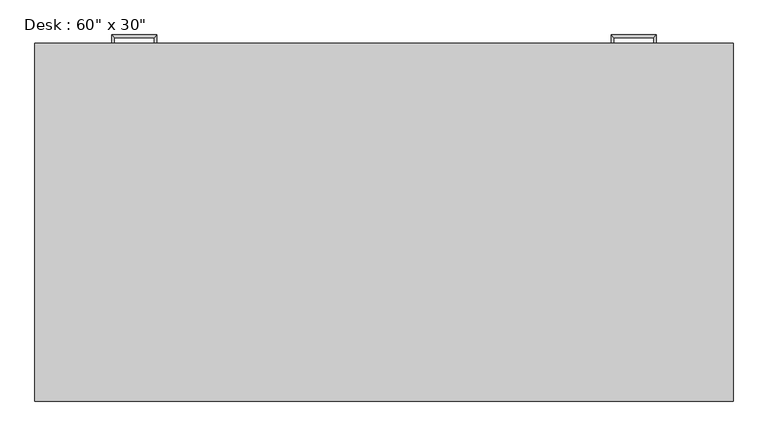
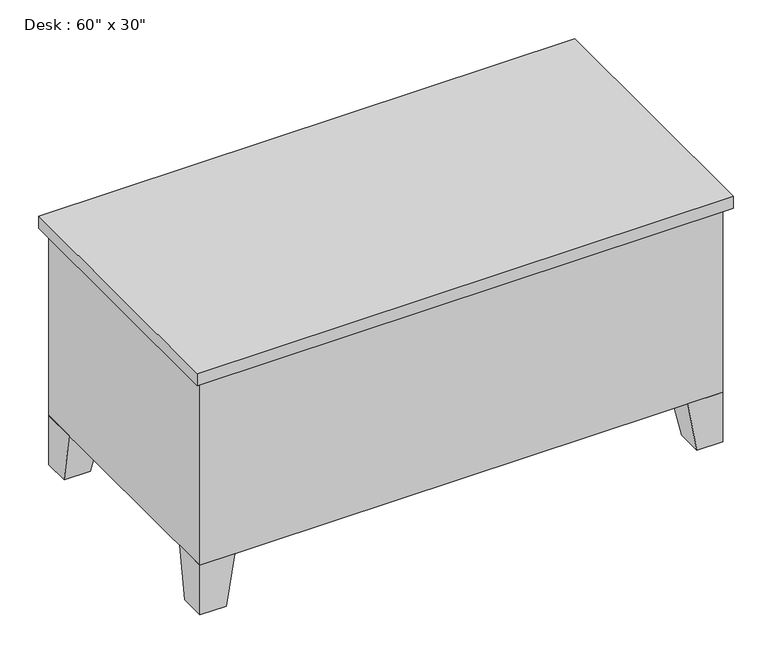
"""IFC4 building model written with IfcOpenShell, lengths in millimetres: furniture geometry."""

import ifcopenshell
import ifcopenshell.guid

model = None  # the IFC model being written
_history = None  # IfcOwnerHistory: only IFC2X3 demands one
_inside = {}  # id of a spatial element -> (the spatial element, [elements in it])
_under = {}  # id of a project, library or spatial element -> (it, [spatial elements below it])
_declared = {}  # id of a project -> (the project, [libraries it declares])
_typed = {}  # id of a type object -> (the type object, [elements of that type])
_made_of = {}  # id of a material, layer set ... -> (it, [elements and type objects made of it])


def new_model(schema):
    """Start an empty IFC model of exactly this schema.

    Asked for "IFC4X3", IfcOpenShell would pick the latest addendum, in which some entities
    have other attributes; the version numbers below select the first issue.
    IFC2X3 requires an IfcOwnerHistory on every rooted entity: one is made here for all.
    """
    global model, _history
    if schema == "IFC4X3":
        model = ifcopenshell.file(schema_version=(4, 3, 0, 0))
    else:
        model = ifcopenshell.file(schema=schema)
    _inside.clear()
    _under.clear()
    _declared.clear()
    _typed.clear()
    _made_of.clear()
    _history = None
    if model.schema == "IFC2X3":
        org = make("IfcOrganization", Name="unknown")
        user = make(
            "IfcPersonAndOrganization",
            ThePerson=make("IfcPerson", FamilyName="unknown"),
            TheOrganization=org,
        )
        app = make(
            "IfcApplication",
            ApplicationDeveloper=org,
            Version="unknown",
            ApplicationFullName="unknown",
            ApplicationIdentifier="unknown",
        )
        _history = make(
            "IfcOwnerHistory",
            OwningUser=user,
            OwningApplication=app,
            ChangeAction="ADDED",
            CreationDate=0,
        )
    return model


def make(cls, **values):
    """One entity of the class cls with the attributes given. An attribute that is None is left unset."""
    return model.create_entity(
        cls, **{name: value for name, value in values.items() if value is not None}
    )


def rooted(cls, **values):
    """An entity with a GlobalId (a new one), such as an element, a storey or a relation."""
    return make(cls, GlobalId=ifcopenshell.guid.new(), OwnerHistory=_history, **values)


def si_unit(unit_type, name, prefix=None):
    """IfcSIUnit, for example si_unit("LENGTHUNIT", "METRE", prefix="MILLI")."""
    return make("IfcSIUnit", UnitType=unit_type, Prefix=prefix, Name=name)


def assignment(units):
    """IfcUnitAssignment: the units of a project."""
    return None if units is None else make("IfcUnitAssignment", Units=units)


def point(xyz):
    """IfcCartesianPoint."""
    return None if xyz is None else make("IfcCartesianPoint", Coordinates=xyz)


def direction(xyz):
    """IfcDirection."""
    return None if xyz is None else make("IfcDirection", DirectionRatios=xyz)


def frame(location, z_axis=None, x_axis=None):
    """IfcAxis2Placement3D, a coordinate frame: its origin and axes. An axis left out is left unset."""
    return make(
        "IfcAxis2Placement3D",
        Location=point(location),
        Axis=direction(z_axis),
        RefDirection=direction(x_axis),
    )


def origin():
    """The frame at (0, 0, 0) with its axes left unset."""
    return frame((0.0, 0.0, 0.0))


def place(relative_to, where):
    """IfcLocalPlacement: puts the frame where relative to a parent placement (None: the world)."""
    return make(
        "IfcLocalPlacement", PlacementRelTo=relative_to, RelativePlacement=where
    )


def context(
    kind, dimensions, precision=None, world=None, true_north=None, identifier=None
):
    """IfcGeometricRepresentationContext, for example the 3D "Model" context."""
    return make(
        "IfcGeometricRepresentationContext",
        ContextIdentifier=identifier,
        ContextType=kind,
        CoordinateSpaceDimension=dimensions,
        Precision=precision,
        WorldCoordinateSystem=world,
        TrueNorth=true_north,
    )


def project(units=None, contexts=None):
    """IfcProject with its units and contexts."""
    return rooted(
        "IfcProject",
        Name="project",
        RepresentationContexts=contexts,
        UnitsInContext=assignment(units),
    )


def spatial(cls, under=None, at=None, **own):
    """A site, building, storey or space (cls), placed at a placement, below another one or the project."""
    s = rooted(cls, ObjectPlacement=at, **own)
    if under is not None:
        _under.setdefault(under.id(), (under, []))[1].append(s)
    return s


def polyline(points):
    """IfcPolyline through the points."""
    return make("IfcPolyline", Points=[point(p) for p in points])


def outline(outer, holes=None, kind="AREA"):
    """IfcArbitraryClosedProfileDef: a profile drawn as a closed curve; with holes, ...WithVoids."""
    if holes is None:
        return make("IfcArbitraryClosedProfileDef", ProfileType=kind, OuterCurve=outer)
    return make(
        "IfcArbitraryProfileDefWithVoids",
        ProfileType=kind,
        OuterCurve=outer,
        InnerCurves=holes,
    )


def extrude(swept, where, along, depth):
    """IfcExtrudedAreaSolid: the profile swept, set in the frame where, extruded along a direction by depth."""
    return make(
        "IfcExtrudedAreaSolid",
        SweptArea=swept,
        Position=where,
        ExtrudedDirection=direction(along),
        Depth=depth,
    )


def faces_of(points, faces, orient=None, outer=None):
    """IfcFace entities. A face is a list of loops; a loop is a list of indices into points, from 0.

    orient and outer hold one flag for each loop. By default every Orientation is true, the
    first loop of a face is its IfcFaceOuterBound and the others are IfcFaceBound.
    """
    made = []
    for i, loops in enumerate(faces):
        bounds = []
        for j, loop in enumerate(loops):
            is_outer = j == 0 if outer is None else outer[i][j]
            bounds.append(
                make(
                    "IfcFaceOuterBound" if is_outer else "IfcFaceBound",
                    Bound=make("IfcPolyLoop", Polygon=[points[k] for k in loop]),
                    Orientation=True if orient is None else orient[i][j],
                )
            )
        made.append(make("IfcFace", Bounds=bounds))
    return made


def faceted_brep(points, faces, orient=None, outer=None, voids=None):
    """IfcFacetedBrep: a solid bounded by flat faces; with voids (closed shells), ...WithVoids."""
    shared = [point(p) for p in points]
    hull = make("IfcClosedShell", CfsFaces=faces_of(shared, faces, orient, outer))
    if voids is None:
        return make("IfcFacetedBrep", Outer=hull)
    return make(
        "IfcFacetedBrepWithVoids",
        Outer=hull,
        Voids=[
            make(cls, CfsFaces=faces_of(shared, fs, o, b)) for cls, fs, o, b in voids
        ],
    )


def shape(context_of_items, identifier, shape_type, items):
    """IfcShapeRepresentation: the items that make up one representation, for example the "Body"."""
    return make(
        "IfcShapeRepresentation",
        ContextOfItems=context_of_items,
        RepresentationIdentifier=identifier,
        RepresentationType=shape_type,
        Items=items,
    )


def source(mapping_origin, context_of_items, identifier, shape_type, items):
    """IfcRepresentationMap: a shape defined once, which mapped items show again and again."""
    return make(
        "IfcRepresentationMap",
        MappingOrigin=mapping_origin,
        MappedRepresentation=shape(context_of_items, identifier, shape_type, items),
    )


def transform(
    local_origin,
    x_axis=None,
    y_axis=None,
    z_axis=None,
    scale=None,
    scale2=None,
    scale3=None,
    uniform=True,
):
    """IfcCartesianTransformationOperator3D, or its non-uniform kind. x_axis, y_axis, z_axis: its Axis1, 2, 3."""
    if uniform:
        return make(
            "IfcCartesianTransformationOperator3D",
            Axis1=direction(x_axis),
            Axis2=direction(y_axis),
            LocalOrigin=point(local_origin),
            Scale=scale,
            Axis3=direction(z_axis),
        )
    return make(
        "IfcCartesianTransformationOperator3DnonUniform",
        Axis1=direction(x_axis),
        Axis2=direction(y_axis),
        LocalOrigin=point(local_origin),
        Scale=scale,
        Axis3=direction(z_axis),
        Scale2=scale2,
        Scale3=scale3,
    )


def mapped(mapping_source, mapping_target):
    """IfcMappedItem: shows the shape of a source again, moved by a transform."""
    return make(
        "IfcMappedItem", MappingSource=mapping_source, MappingTarget=mapping_target
    )


def made_of(thing, what):
    """Note that an element or type object is made of a material, layer set ...; save() writes the relation."""
    if what is not None:
        _made_of.setdefault(what.id(), (what, []))[1].append(thing)
    return thing


def element(
    cls,
    number,
    at=None,
    inside=None,
    cuts=None,
    type_object=None,
    material=None,
    context=None,
    identifier="Body",
    shape_type=None,
    held_by="IfcProductDefinitionShape",
    body=None,
    shapes=None,
    **own,
):
    """One element of the class cls, such as IfcWall. Its Tag is "e" and its number.

    at: its placement. inside: the storey or other place that contains it. cuts: it is an
    opening in that element (IfcRelVoidsElement). A single representation is given by context,
    identifier, shape_type and body (its items); several are given by shapes. held_by: the class
    of the entity that holds the representations. save() writes the other relations.
    """
    e = rooted(cls, Tag="e%d" % number, ObjectPlacement=at, **own)
    if body is not None:
        shapes = [shape(context, identifier, shape_type, body)]
    if shapes is not None:
        e.Representation = make(held_by, Representations=shapes)
    if inside is not None:
        _inside.setdefault(inside.id(), (inside, []))[1].append(e)
    if cuts is not None:
        rooted(
            "IfcRelVoidsElement", RelatingBuildingElement=cuts, RelatedOpeningElement=e
        )
    if type_object is not None:
        _typed.setdefault(type_object.id(), (type_object, []))[1].append(e)
    return made_of(e, material)


def aggregate(whole, parts):
    """IfcRelAggregates: a whole, such as a stair, and the parts it consists of."""
    return rooted("IfcRelAggregates", RelatingObject=whole, RelatedObjects=parts)


def save(model, path):
    """Write the relations noted so far, then the file.

    IfcRelAggregates (storeys below a building ...), IfcRelContainedInSpatialStructure (elements
    in a storey), IfcRelDefinesByType, IfcRelAssociatesMaterial and IfcRelDeclares: one each for
    every whole, place, type object, material and project.
    """
    for whole, parts in _under.values():
        aggregate(whole, parts)
    for where, things in _inside.values():
        rooted(
            "IfcRelContainedInSpatialStructure",
            RelatedElements=things,
            RelatingStructure=where,
        )
    for kind, things in _typed.values():
        rooted("IfcRelDefinesByType", RelatedObjects=things, RelatingType=kind)
    for what, things in _made_of.values():
        rooted("IfcRelAssociatesMaterial", RelatedObjects=things, RelatingMaterial=what)
    for by, libraries in _declared.values():
        rooted("IfcRelDeclares", RelatingContext=by, RelatedDefinitions=libraries)
    model.write(path)


def furniture_072f6425(model_context):
    return source(origin(), model_context, "Body", "SolidModel", [
        extrude(outline(polyline([(1504.95, 762.0), (1136.65, 762.0), (1136.65, 774.7), (1504.95, 774.7), (1504.95, 762.0)])), frame((0.0, 0.0, 603.25), z_axis=(0.0, 0.0, 1.0), x_axis=(1.0, 0.0, 0.0)), (0.0, 0.0, 1.0), 101.6),
        extrude(outline(polyline([(1504.95, 762.0), (1136.65, 762.0), (1136.65, 774.7), (1504.95, 774.7), (1504.95, 762.0)])), frame((0.0, 0.0, 171.45), z_axis=(0.0, 0.0, 1.0), x_axis=(1.0, 0.0, 0.0)), (0.0, 0.0, 1.0), 412.75),
        extrude(outline(polyline([(387.35, 762.0), (19.05, 762.0), (19.05, 774.7), (387.35, 774.7), (387.35, 762.0)])), frame((0.0, 0.0, 603.25), z_axis=(0.0, 0.0, 1.0), x_axis=(1.0, 0.0, 0.0)), (0.0, 0.0, 1.0), 101.6),
        extrude(outline(polyline([(387.35, 762.0), (19.05, 762.0), (19.05, 774.7), (387.35, 774.7), (387.35, 762.0)])), frame((0.0, 0.0, 171.45), z_axis=(0.0, 0.0, 1.0), x_axis=(1.0, 0.0, 0.0)), (0.0, 0.0, 1.0), 171.45),
        extrude(outline(polyline([(387.35, 762.0), (19.05, 762.0), (19.05, 774.7), (387.35, 774.7), (387.35, 762.0)])), frame((0.0, 0.0, 482.6), z_axis=(0.0, 0.0, 1.0), x_axis=(1.0, 0.0, 0.0)), (0.0, 0.0, 1.0), 101.6),
        extrude(outline(polyline([(387.35, 762.0), (19.05, 762.0), (19.05, 774.7), (387.35, 774.7), (387.35, 762.0)])), frame((0.0, 0.0, 361.95), z_axis=(0.0, 0.0, 1.0), x_axis=(1.0, 0.0, 0.0)), (0.0, 0.0, 1.0), 101.6),
        faceted_brep([(1422.4, 762.0, 152.4), (1422.4, 660.4, 152.4), (1524.0, 660.4, 152.4), (1524.0, 762.0, 152.4), (1447.8, 762.0, 0.0), (1524.0, 762.0, 0.0), (1524.0, 685.8, 0.0), (1447.8, 685.8, 0.0)], [[[0, 1, 2, 3]], [[4, 5, 6, 7]], [[4, 7, 1, 0]], [[7, 6, 2, 1]], [[6, 5, 3, 2]], [[5, 4, 0, 3]]]),
        faceted_brep([(1422.4, 0.0, 152.4), (1524.0, 0.0, 152.4), (1524.0, 101.6, 152.4), (1422.4, 101.6, 152.4), (1447.8, 0.0, 0.0), (1447.8, 76.2, 0.0), (1524.0, 76.2, 0.0), (1524.0, 0.0, 0.0)], [[[0, 1, 2, 3]], [[4, 5, 6, 7]], [[4, 7, 1, 0]], [[7, 6, 2, 1]], [[6, 5, 3, 2]], [[5, 4, 0, 3]]]),
        faceted_brep([(101.6, 0.0, 152.4), (101.6, 101.6, 152.4), (0.0, 101.6, 152.4), (0.0, 0.0, 152.4), (76.2, 0.0, 0.0), (0.0, 0.0, 0.0), (0.0, 76.2, 0.0), (76.2, 76.2, 0.0)], [[[0, 1, 2, 3]], [[4, 5, 6, 7]], [[4, 7, 1, 0]], [[7, 6, 2, 1]], [[6, 5, 3, 2]], [[5, 4, 0, 3]]]),
        faceted_brep([(101.6, 762.0, 152.4), (0.0, 762.0, 152.4), (0.0, 660.4, 152.4), (101.6, 660.4, 152.4), (76.2, 762.0, 0.0), (76.2, 685.8, 0.0), (0.0, 685.8, 0.0), (0.0, 762.0, 0.0)], [[[0, 1, 2, 3]], [[4, 5, 6, 7]], [[4, 7, 1, 0]], [[7, 6, 2, 1]], [[6, 5, 3, 2]], [[5, 4, 0, 3]]]),
        extrude(outline(polyline([(1543.05, 781.05), (1543.05, -19.05), (-19.05, -19.05), (-19.05, 781.05), (1543.05, 781.05)])), frame((0.0, 0.0, 723.9), z_axis=(0.0, 0.0, 1.0), x_axis=(1.0, 0.0, 0.0)), (0.0, 0.0, 1.0), 38.1),
        extrude(outline(polyline([(406.4, 762.0), (406.4, 50.8), (1117.6, 50.8), (1117.6, 762.0), (1524.0, 762.0), (1524.0, 0.0), (0.0, 0.0), (0.0, 762.0), (406.4, 762.0)])), frame((0.0, 0.0, 152.4), z_axis=(0.0, 0.0, 1.0), x_axis=(1.0, 0.0, 0.0)), (0.0, 0.0, 1.0), 571.5),
        faceted_brep([(1365.25, 774.7, 546.1), (1365.25, 774.7, 533.4), (1371.6, 774.7, 533.4), (1371.6, 774.7, 546.1), (1365.25, 793.75, 546.1), (1365.25, 793.75, 533.4), (1371.6, 800.1, 533.4), (1371.6, 800.1, 546.1), (1276.35, 793.75, 546.1), (1276.35, 793.75, 533.4), (1270.0, 800.1, 533.4), (1270.0, 800.1, 546.1), (1276.35, 774.7, 546.1), (1270.0, 774.7, 546.1), (1270.0, 774.7, 533.4), (1276.35, 774.7, 533.4)], [[[0, 1, 2, 3]], [[1, 0, 4, 5]], [[2, 1, 5, 6]], [[3, 2, 6, 7]], [[0, 3, 7, 4]], [[5, 4, 8, 9]], [[6, 5, 9, 10]], [[7, 6, 10, 11]], [[4, 7, 11, 8]], [[12, 13, 14, 15]], [[9, 8, 12, 15]], [[10, 9, 15, 14]], [[11, 10, 14, 13]], [[8, 11, 13, 12]]]),
        faceted_brep([(1365.25, 774.7, 666.75), (1365.25, 774.7, 654.05), (1371.6, 774.7, 654.05), (1371.6, 774.7, 666.75), (1365.25, 793.75, 666.75), (1365.25, 793.75, 654.05), (1371.6, 800.1, 654.05), (1371.6, 800.1, 666.75), (1276.35, 793.75, 666.75), (1276.35, 793.75, 654.05), (1270.0, 800.1, 654.05), (1270.0, 800.1, 666.75), (1276.35, 774.7, 666.75), (1270.0, 774.7, 666.75), (1270.0, 774.7, 654.05), (1276.35, 774.7, 654.05)], [[[0, 1, 2, 3]], [[1, 0, 4, 5]], [[2, 1, 5, 6]], [[3, 2, 6, 7]], [[0, 3, 7, 4]], [[5, 4, 8, 9]], [[6, 5, 9, 10]], [[7, 6, 10, 11]], [[4, 7, 11, 8]], [[12, 13, 14, 15]], [[9, 8, 12, 15]], [[10, 9, 15, 14]], [[11, 10, 14, 13]], [[8, 11, 13, 12]]]),
        faceted_brep([(158.75, 774.7, 304.8), (152.4, 774.7, 304.8), (152.4, 774.7, 292.1), (158.75, 774.7, 292.1), (158.75, 793.75, 304.8), (152.4, 800.1, 304.8), (152.4, 800.1, 292.1), (158.75, 793.75, 292.1), (247.65, 793.75, 304.8), (254.0, 800.1, 304.8), (254.0, 800.1, 292.1), (247.65, 793.75, 292.1), (247.65, 774.7, 304.8), (247.65, 774.7, 292.1), (254.0, 774.7, 292.1), (254.0, 774.7, 304.8)], [[[0, 1, 2, 3]], [[1, 0, 4, 5]], [[2, 1, 5, 6]], [[3, 2, 6, 7]], [[0, 3, 7, 4]], [[5, 4, 8, 9]], [[6, 5, 9, 10]], [[7, 6, 10, 11]], [[4, 7, 11, 8]], [[12, 13, 14, 15]], [[9, 8, 12, 15]], [[10, 9, 15, 14]], [[11, 10, 14, 13]], [[8, 11, 13, 12]]]),
        faceted_brep([(158.75, 774.7, 425.45), (152.4, 774.7, 425.45), (152.4, 774.7, 412.75), (158.75, 774.7, 412.75), (158.75, 793.75, 425.45), (152.4, 800.1, 425.45), (152.4, 800.1, 412.75), (158.75, 793.75, 412.75), (247.65, 793.75, 425.45), (254.0, 800.1, 425.45), (254.0, 800.1, 412.75), (247.65, 793.75, 412.75), (247.65, 774.7, 425.45), (247.65, 774.7, 412.75), (254.0, 774.7, 412.75), (254.0, 774.7, 425.45)], [[[0, 1, 2, 3]], [[1, 0, 4, 5]], [[2, 1, 5, 6]], [[3, 2, 6, 7]], [[0, 3, 7, 4]], [[5, 4, 8, 9]], [[6, 5, 9, 10]], [[7, 6, 10, 11]], [[4, 7, 11, 8]], [[12, 13, 14, 15]], [[9, 8, 12, 15]], [[10, 9, 15, 14]], [[11, 10, 14, 13]], [[8, 11, 13, 12]]]),
        faceted_brep([(158.75, 774.7, 546.1), (152.4, 774.7, 546.1), (152.4, 774.7, 533.4), (158.75, 774.7, 533.4), (158.75, 793.75, 546.1), (152.4, 800.1, 546.1), (152.4, 800.1, 533.4), (158.75, 793.75, 533.4), (247.65, 793.75, 546.1), (254.0, 800.1, 546.1), (254.0, 800.1, 533.4), (247.65, 793.75, 533.4), (247.65, 774.7, 546.1), (247.65, 774.7, 533.4), (254.0, 774.7, 533.4), (254.0, 774.7, 546.1)], [[[0, 1, 2, 3]], [[1, 0, 4, 5]], [[2, 1, 5, 6]], [[3, 2, 6, 7]], [[0, 3, 7, 4]], [[5, 4, 8, 9]], [[6, 5, 9, 10]], [[7, 6, 10, 11]], [[4, 7, 11, 8]], [[12, 13, 14, 15]], [[9, 8, 12, 15]], [[10, 9, 15, 14]], [[11, 10, 14, 13]], [[8, 11, 13, 12]]]),
        faceted_brep([(158.75, 774.7, 666.75), (152.4, 774.7, 666.75), (152.4, 774.7, 654.05), (158.75, 774.7, 654.05), (158.75, 793.75, 666.75), (152.4, 800.1, 666.75), (152.4, 800.1, 654.05), (158.75, 793.75, 654.05), (247.65, 793.75, 666.75), (254.0, 800.1, 666.75), (254.0, 800.1, 654.05), (247.65, 793.75, 654.05), (247.65, 774.7, 666.75), (247.65, 774.7, 654.05), (254.0, 774.7, 654.05), (254.0, 774.7, 666.75)], [[[0, 1, 2, 3]], [[1, 0, 4, 5]], [[2, 1, 5, 6]], [[3, 2, 6, 7]], [[0, 3, 7, 4]], [[5, 4, 8, 9]], [[6, 5, 9, 10]], [[7, 6, 10, 11]], [[4, 7, 11, 8]], [[12, 13, 14, 15]], [[9, 8, 12, 15]], [[10, 9, 15, 14]], [[11, 10, 14, 13]], [[8, 11, 13, 12]]]),
    ])


if __name__ == "__main__":
    model = new_model("IFC4")
    model_context = context("Model", 3, world=origin())
    ifc_project = project(units=[si_unit("LENGTHUNIT", "METRE", prefix="MILLI")], contexts=[model_context])
    site = spatial("IfcSite", under=ifc_project)
    building = spatial("IfcBuilding", under=site)
    placement = place(None, origin())
    furniture_shape = furniture_072f6425(model_context)
    element("IfcFurniture", 1, ObjectType="Desk : 60\" x 30\"", at=placement, inside=building, context=model_context, shape_type="MappedRepresentation", body=[
        mapped(furniture_shape, transform((0.0, 0.0, 0.0), x_axis=(1.0, 0.0, 0.0), y_axis=(0.0, 1.0, 0.0), z_axis=(0.0, 0.0, 1.0))),
    ])
    save(model, "model.ifc")

# Revit data of these elements
# Project information
#   Project Issue Date = "Issue Date"
#   Project Status = "Project Status"
#   Client Name = "Owner"
#   Project Address = "Enter address here"
#   Project Name = "Project Name"
#   Project Number = "Project Number"
# Type "Desk : 60\" x 30\""
#   Assembly Code = "E2020200"
#   Depth = 2' - 6"
#   Height = 2' - 6"
#   Leg Height = 0' - 6"
#   Width = 5' - 0"
#   Body Material = Laminate, Ivory, Matte
#   Handle/Leg Material = Steel, Chrome Plated
#   Top Material = Cherry
#   Default Elevation = 0
# Element 1 (IfcFurniture, "Desk : 60\" x 30\"")
#   Materials on its faces: "Steel, Chrome Plated", "Laminate, Ivory, Matte", "Cherry"
# Materials
#   "Laminate, Ivory, Matte": class "Plastic", colour RGB 247 247 239, transparency 0, Description = "Plastic Laminate - Ivory, Matte", Cost = 0
#   "Steel, Chrome Plated": class "Metal", colour RGB 17 17 17, transparency 0, Description = "Chromiuim plated steel", Cost = 0
#   "Cherry": class "Wood", colour RGB 226 177 128, transparency 0, Description = "Prunus Serotina", Cost = 0
